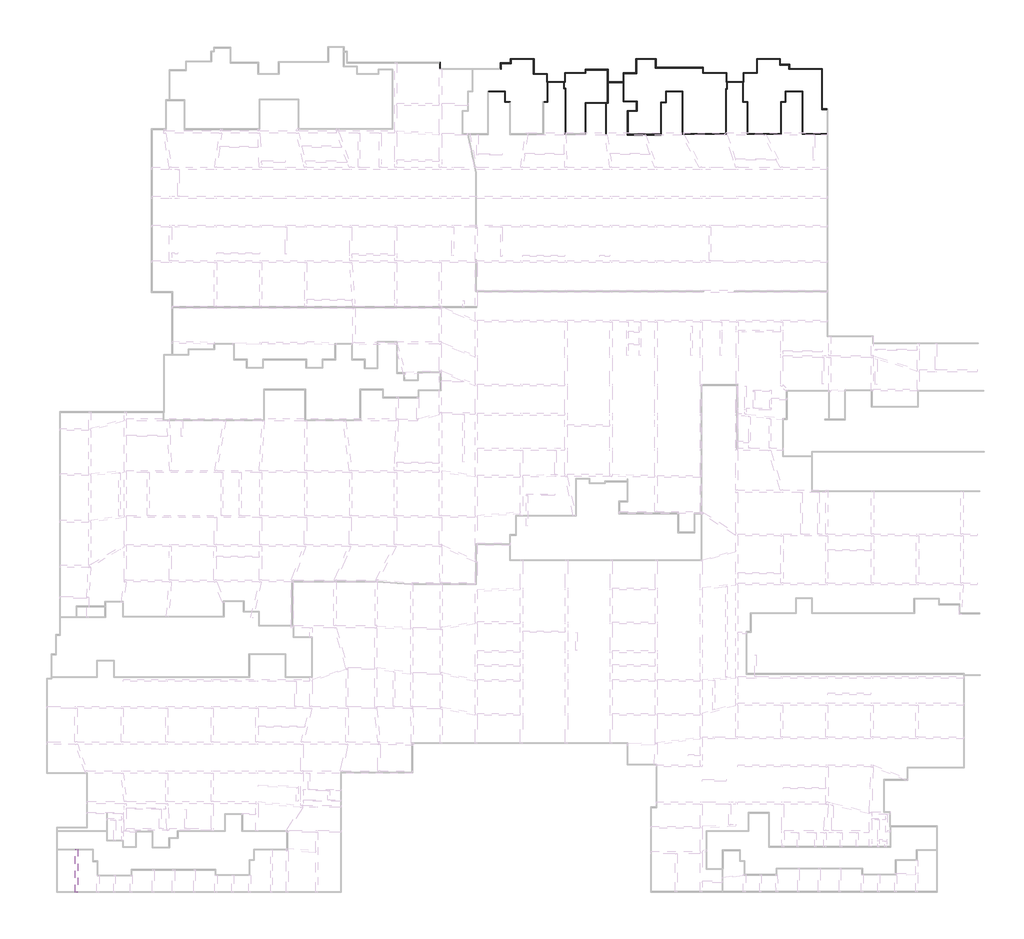
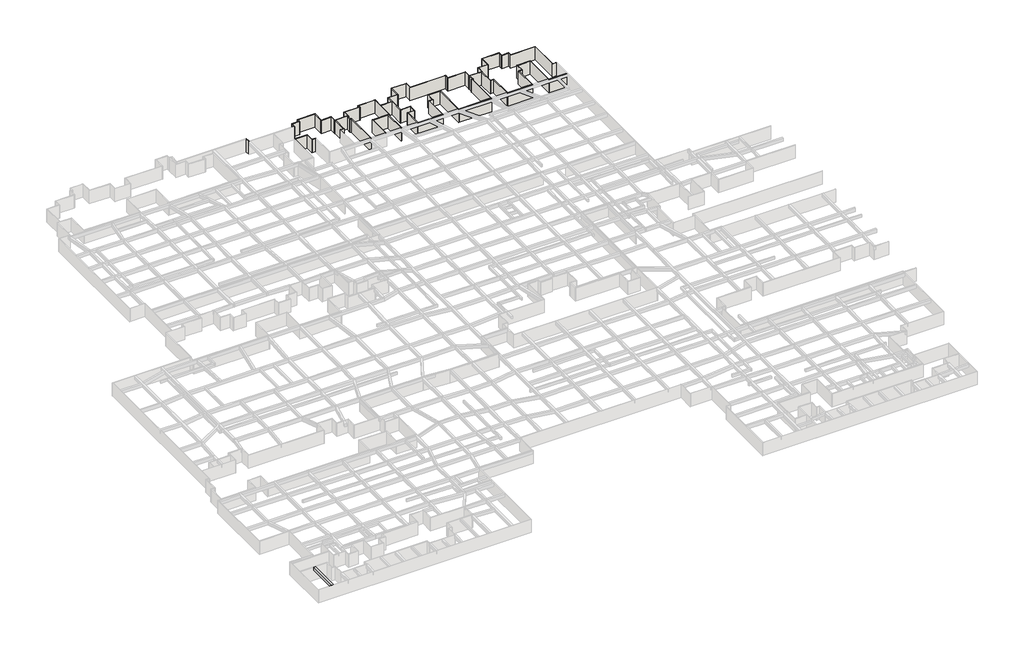
# One storey, part 5 of 16: 70 walls, 1 beam.
"""IFC4 building model written with IfcOpenShell, lengths in millimetres."""

import ifcopenshell
import ifcopenshell.guid

model = None  # the IFC model being written
_history = None  # IfcOwnerHistory: only IFC2X3 demands one
_inside = {}  # id of a spatial element -> (the spatial element, [elements in it])
_under = {}  # id of a project, library or spatial element -> (it, [spatial elements below it])
_declared = {}  # id of a project -> (the project, [libraries it declares])
_typed = {}  # id of a type object -> (the type object, [elements of that type])
_made_of = {}  # id of a material, layer set ... -> (it, [elements and type objects made of it])


def new_model(schema):
    """Start an empty IFC model of exactly this schema.

    Asked for "IFC4X3", IfcOpenShell would pick the latest addendum, in which some entities
    have other attributes; the version numbers below select the first issue.
    IFC2X3 requires an IfcOwnerHistory on every rooted entity: one is made here for all.
    """
    global model, _history
    if schema == "IFC4X3":
        model = ifcopenshell.file(schema_version=(4, 3, 0, 0))
    else:
        model = ifcopenshell.file(schema=schema)
    _inside.clear()
    _under.clear()
    _declared.clear()
    _typed.clear()
    _made_of.clear()
    _history = None
    if model.schema == "IFC2X3":
        org = make("IfcOrganization", Name="unknown")
        user = make(
            "IfcPersonAndOrganization",
            ThePerson=make("IfcPerson", FamilyName="unknown"),
            TheOrganization=org,
        )
        app = make(
            "IfcApplication",
            ApplicationDeveloper=org,
            Version="unknown",
            ApplicationFullName="unknown",
            ApplicationIdentifier="unknown",
        )
        _history = make(
            "IfcOwnerHistory",
            OwningUser=user,
            OwningApplication=app,
            ChangeAction="ADDED",
            CreationDate=0,
        )
    return model


def make(cls, **values):
    """One entity of the class cls with the attributes given. An attribute that is None is left unset."""
    return model.create_entity(
        cls, **{name: value for name, value in values.items() if value is not None}
    )


def rooted(cls, **values):
    """An entity with a GlobalId (a new one), such as an element, a storey or a relation."""
    return make(cls, GlobalId=ifcopenshell.guid.new(), OwnerHistory=_history, **values)


def si_unit(unit_type, name, prefix=None):
    """IfcSIUnit, for example si_unit("LENGTHUNIT", "METRE", prefix="MILLI")."""
    return make("IfcSIUnit", UnitType=unit_type, Prefix=prefix, Name=name)


def assignment(units):
    """IfcUnitAssignment: the units of a project."""
    return None if units is None else make("IfcUnitAssignment", Units=units)


def point(xyz):
    """IfcCartesianPoint."""
    return None if xyz is None else make("IfcCartesianPoint", Coordinates=xyz)


def direction(xyz):
    """IfcDirection."""
    return None if xyz is None else make("IfcDirection", DirectionRatios=xyz)


def frame(location, z_axis=None, x_axis=None):
    """IfcAxis2Placement3D, a coordinate frame: its origin and axes. An axis left out is left unset."""
    return make(
        "IfcAxis2Placement3D",
        Location=point(location),
        Axis=direction(z_axis),
        RefDirection=direction(x_axis),
    )


def origin():
    """The frame at (0, 0, 0) with its axes left unset."""
    return frame((0.0, 0.0, 0.0))


def origin_with_axes():
    """The frame at (0, 0, 0) with the z axis (0, 0, 1) and the x axis (1, 0, 0) written out."""
    return frame((0.0, 0.0, 0.0), z_axis=(0.0, 0.0, 1.0), x_axis=(1.0, 0.0, 0.0))


def place(relative_to, where):
    """IfcLocalPlacement: puts the frame where relative to a parent placement (None: the world)."""
    return make(
        "IfcLocalPlacement", PlacementRelTo=relative_to, RelativePlacement=where
    )


def context(
    kind, dimensions, precision=None, world=None, true_north=None, identifier=None
):
    """IfcGeometricRepresentationContext, for example the 3D "Model" context."""
    return make(
        "IfcGeometricRepresentationContext",
        ContextIdentifier=identifier,
        ContextType=kind,
        CoordinateSpaceDimension=dimensions,
        Precision=precision,
        WorldCoordinateSystem=world,
        TrueNorth=true_north,
    )


def project(units=None, contexts=None):
    """IfcProject with its units and contexts."""
    return rooted(
        "IfcProject",
        Name="project",
        RepresentationContexts=contexts,
        UnitsInContext=assignment(units),
    )


def spatial(cls, under=None, at=None, **own):
    """A site, building, storey or space (cls), placed at a placement, below another one or the project."""
    s = rooted(cls, ObjectPlacement=at, **own)
    if under is not None:
        _under.setdefault(under.id(), (under, []))[1].append(s)
    return s


def polyline(points):
    """IfcPolyline through the points."""
    return make("IfcPolyline", Points=[point(p) for p in points])


def outline(outer, holes=None, kind="AREA"):
    """IfcArbitraryClosedProfileDef: a profile drawn as a closed curve; with holes, ...WithVoids."""
    if holes is None:
        return make("IfcArbitraryClosedProfileDef", ProfileType=kind, OuterCurve=outer)
    return make(
        "IfcArbitraryProfileDefWithVoids",
        ProfileType=kind,
        OuterCurve=outer,
        InnerCurves=holes,
    )


def extrude(swept, where, along, depth):
    """IfcExtrudedAreaSolid: the profile swept, set in the frame where, extruded along a direction by depth."""
    return make(
        "IfcExtrudedAreaSolid",
        SweptArea=swept,
        Position=where,
        ExtrudedDirection=direction(along),
        Depth=depth,
    )


def faces_of(points, faces, orient=None, outer=None):
    """IfcFace entities. A face is a list of loops; a loop is a list of indices into points, from 0.

    orient and outer hold one flag for each loop. By default every Orientation is true, the
    first loop of a face is its IfcFaceOuterBound and the others are IfcFaceBound.
    """
    made = []
    for i, loops in enumerate(faces):
        bounds = []
        for j, loop in enumerate(loops):
            is_outer = j == 0 if outer is None else outer[i][j]
            bounds.append(
                make(
                    "IfcFaceOuterBound" if is_outer else "IfcFaceBound",
                    Bound=make("IfcPolyLoop", Polygon=[points[k] for k in loop]),
                    Orientation=True if orient is None else orient[i][j],
                )
            )
        made.append(make("IfcFace", Bounds=bounds))
    return made


def faceted_brep(points, faces, orient=None, outer=None, voids=None):
    """IfcFacetedBrep: a solid bounded by flat faces; with voids (closed shells), ...WithVoids."""
    shared = [point(p) for p in points]
    hull = make("IfcClosedShell", CfsFaces=faces_of(shared, faces, orient, outer))
    if voids is None:
        return make("IfcFacetedBrep", Outer=hull)
    return make(
        "IfcFacetedBrepWithVoids",
        Outer=hull,
        Voids=[
            make(cls, CfsFaces=faces_of(shared, fs, o, b)) for cls, fs, o, b in voids
        ],
    )


def shape(context_of_items, identifier, shape_type, items):
    """IfcShapeRepresentation: the items that make up one representation, for example the "Body"."""
    return make(
        "IfcShapeRepresentation",
        ContextOfItems=context_of_items,
        RepresentationIdentifier=identifier,
        RepresentationType=shape_type,
        Items=items,
    )


def source(mapping_origin, context_of_items, identifier, shape_type, items):
    """IfcRepresentationMap: a shape defined once, which mapped items show again and again."""
    return make(
        "IfcRepresentationMap",
        MappingOrigin=mapping_origin,
        MappedRepresentation=shape(context_of_items, identifier, shape_type, items),
    )


def transform(
    local_origin,
    x_axis=None,
    y_axis=None,
    z_axis=None,
    scale=None,
    scale2=None,
    scale3=None,
    uniform=True,
):
    """IfcCartesianTransformationOperator3D, or its non-uniform kind. x_axis, y_axis, z_axis: its Axis1, 2, 3."""
    if uniform:
        return make(
            "IfcCartesianTransformationOperator3D",
            Axis1=direction(x_axis),
            Axis2=direction(y_axis),
            LocalOrigin=point(local_origin),
            Scale=scale,
            Axis3=direction(z_axis),
        )
    return make(
        "IfcCartesianTransformationOperator3DnonUniform",
        Axis1=direction(x_axis),
        Axis2=direction(y_axis),
        LocalOrigin=point(local_origin),
        Scale=scale,
        Axis3=direction(z_axis),
        Scale2=scale2,
        Scale3=scale3,
    )


def mapped(mapping_source, mapping_target):
    """IfcMappedItem: shows the shape of a source again, moved by a transform."""
    return make(
        "IfcMappedItem", MappingSource=mapping_source, MappingTarget=mapping_target
    )


def made_of(thing, what):
    """Note that an element or type object is made of a material, layer set ...; save() writes the relation."""
    if what is not None:
        _made_of.setdefault(what.id(), (what, []))[1].append(thing)
    return thing


def element(
    cls,
    number,
    at=None,
    inside=None,
    cuts=None,
    type_object=None,
    material=None,
    context=None,
    identifier="Body",
    shape_type=None,
    held_by="IfcProductDefinitionShape",
    body=None,
    shapes=None,
    **own,
):
    """One element of the class cls, such as IfcWall. Its Tag is "e" and its number.

    at: its placement. inside: the storey or other place that contains it. cuts: it is an
    opening in that element (IfcRelVoidsElement). A single representation is given by context,
    identifier, shape_type and body (its items); several are given by shapes. held_by: the class
    of the entity that holds the representations. save() writes the other relations.
    """
    e = rooted(cls, Tag="e%d" % number, ObjectPlacement=at, **own)
    if body is not None:
        shapes = [shape(context, identifier, shape_type, body)]
    if shapes is not None:
        e.Representation = make(held_by, Representations=shapes)
    if inside is not None:
        _inside.setdefault(inside.id(), (inside, []))[1].append(e)
    if cuts is not None:
        rooted(
            "IfcRelVoidsElement", RelatingBuildingElement=cuts, RelatedOpeningElement=e
        )
    if type_object is not None:
        _typed.setdefault(type_object.id(), (type_object, []))[1].append(e)
    return made_of(e, material)


def aggregate(whole, parts):
    """IfcRelAggregates: a whole, such as a stair, and the parts it consists of."""
    return rooted("IfcRelAggregates", RelatingObject=whole, RelatedObjects=parts)


def save(model, path):
    """Write the relations noted so far, then the file.

    IfcRelAggregates (storeys below a building ...), IfcRelContainedInSpatialStructure (elements
    in a storey), IfcRelDefinesByType, IfcRelAssociatesMaterial and IfcRelDeclares: one each for
    every whole, place, type object, material and project.
    """
    for whole, parts in _under.values():
        aggregate(whole, parts)
    for where, things in _inside.values():
        rooted(
            "IfcRelContainedInSpatialStructure",
            RelatedElements=things,
            RelatingStructure=where,
        )
    for kind, things in _typed.values():
        rooted("IfcRelDefinesByType", RelatedObjects=things, RelatingType=kind)
    for what, things in _made_of.values():
        rooted("IfcRelAssociatesMaterial", RelatedObjects=things, RelatingMaterial=what)
    for by, libraries in _declared.values():
        rooted("IfcRelDeclares", RelatingContext=by, RelatedDefinitions=libraries)
    model.write(path)


def kl_beam_eab3c69a(model_context):
    return source(origin(), model_context, "Body", "SweptSolid", [
        extrude(outline(polyline([(3851.0, 200.0), (3851.0, -200.0), (-3851.0, -200.0), (-3851.0, 200.0), (3851.0, 200.0)])), frame((0.0, 0.0, -400.0), z_axis=(0.0, 0.0, 1.0), x_axis=(1.0, 0.0, 0.0)), (0.0, 0.0, 1.0), 800.0),
    ])


model = new_model("IFC4")

# Units and contexts
model_context = context("Model", 3, world=origin())
ifc_project = project(units=[si_unit("LENGTHUNIT", "METRE", prefix="MILLI")], contexts=[model_context])

# Site, building, storey
site = spatial("IfcSite", under=ifc_project)
building = spatial("IfcBuilding", under=site)
storey = spatial("IfcBuildingStorey", under=building, Name="户型图", Elevation=0.0)

# Beam
placement = place(None, origin())
kl_beam_shape = kl_beam_eab3c69a(model_context)
element("IfcBeam", 1, ObjectType="KL_beam", at=placement, inside=storey, context=model_context, shape_type="MappedRepresentation", body=[
    mapped(kl_beam_shape, transform((69597.2422757, 63756.0820134, 2900.0), x_axis=(0.0, 1.0, 0.0), y_axis=(-1.0, 0.0, 0.0), z_axis=(0.0, 0.0, 1.0))),
])

# Walls
element("IfcWall", 2, at=placement, inside=storey, context=model_context, shape_type="Brep", body=[
    faceted_brep([(204566.5546537, 200822.7290951, 0.0), (203726.5546537, 200822.7290951, 0.0), (203606.5546537, 200822.7290951, 0.0), (203606.5546537, 200822.7290951, 3300.0), (203726.5546537, 200822.7290951, 3300.0), (204566.5546537, 200822.7290951, 3300.0), (204566.5546537, 200702.7290951, 0.0), (204566.5546537, 200702.7290951, 3300.0), (203606.5546537, 200702.7290951, 3300.0), (203606.5546537, 200702.7290951, 0.0)], [[[0, 1, 2, 3, 4, 5]], [[6, 7, 8, 9]], [[2, 1, 0, 6, 9]], [[5, 4, 3, 8, 7]], [[0, 5, 7, 6]], [[3, 2, 9, 8]]]),
])
element("IfcWall", 3, at=placement, inside=storey, context=model_context, shape_type="Brep", body=[
    faceted_brep([(203726.5546537, 200822.7290951, 0.0), (203726.5546537, 208022.6509701, 0.0), (203726.5546537, 208022.6509701, 3300.0), (203726.5546537, 200822.7290951, 3300.0), (203606.5546537, 200822.7290951, 0.0), (203606.5546537, 200822.7290951, 3300.0), (203606.5546537, 207902.6509701, 3300.0), (203606.5546537, 208022.6509701, 3300.0), (203606.5546537, 208022.6509701, 0.0), (203606.5546537, 207902.6509701, 0.0)], [[[0, 1, 2, 3]], [[4, 5, 6, 7, 8, 9]], [[1, 0, 4, 9, 8]], [[3, 2, 7, 6, 5]], [[0, 3, 5, 4]], [[2, 1, 8, 7]]]),
])
element("IfcWall", 4, at=placement, inside=storey, context=model_context, shape_type="Brep", body=[
    faceted_brep([(203606.5546537, 208022.6509701, 0.0), (197813.5060859, 208022.6509701, 0.0), (197693.5060859, 208022.6509701, 0.0), (197693.5060859, 208022.6509701, 3300.0), (197813.5060859, 208022.6509701, 3300.0), (203606.5546537, 208022.6509701, 3300.0), (203606.5546537, 207902.6509701, 0.0), (203606.5546537, 207902.6509701, 3300.0), (197693.5060859, 207902.6509701, 3300.0), (197693.5060859, 207902.6509701, 0.0)], [[[0, 1, 2, 3, 4, 5]], [[6, 7, 8, 9]], [[2, 1, 0, 6, 9]], [[5, 4, 3, 8, 7]], [[0, 5, 7, 6]], [[3, 2, 9, 8]]]),
])
element("IfcWall", 5, at=placement, inside=storey, context=model_context, shape_type="Brep", body=[
    faceted_brep([(197813.5060859, 208022.6509701, 0.0), (197813.5060859, 208822.5710733, 0.0), (197813.5060859, 208822.5710733, 3300.0), (197813.5060859, 208022.6509701, 3300.0), (197693.5060859, 208022.6509701, 0.0), (197693.5060859, 208022.6509701, 3300.0), (197693.5060859, 208702.5710733, 3300.0), (197693.5060859, 208822.5710733, 3300.0), (197693.5060859, 208822.5710733, 0.0), (197693.5060859, 208702.5710733, 0.0)], [[[0, 1, 2, 3]], [[4, 5, 6, 7, 8, 9]], [[1, 0, 4, 9, 8]], [[3, 2, 7, 6, 5]], [[0, 3, 5, 4]], [[2, 1, 8, 7]]]),
])
element("IfcWall", 6, at=placement, inside=storey, context=model_context, shape_type="Brep", body=[
    faceted_brep([(197693.5060859, 208822.5710733, 0.0), (196163.5308894, 208822.5710733, 0.0), (196043.5308894, 208822.5710733, 0.0), (196043.5308894, 208822.5710733, 3300.0), (196163.5308894, 208822.5710733, 3300.0), (197693.5060859, 208822.5710733, 3300.0), (197693.5060859, 208702.5710733, 0.0), (197693.5060859, 208702.5710733, 3300.0), (196043.5308894, 208702.5710733, 3300.0), (196043.5308894, 208702.5710733, 0.0)], [[[0, 1, 2, 3, 4, 5]], [[6, 7, 8, 9]], [[2, 1, 0, 6, 9]], [[5, 4, 3, 8, 7]], [[0, 5, 7, 6]], [[3, 2, 9, 8]]]),
])
element("IfcWall", 7, at=placement, inside=storey, context=model_context, shape_type="Brep", body=[
    faceted_brep([(196163.5308894, 208822.5710733, 0.0), (196163.5308894, 209822.6499935, 0.0), (196163.5308894, 209822.6499935, 3300.0), (196163.5308894, 208822.5710733, 3300.0), (196043.5308894, 208822.5710733, 0.0), (196043.5308894, 208822.5710733, 3300.0), (196043.5308894, 209702.6499935, 3300.0), (196043.5308894, 209822.6499935, 3300.0), (196043.5308894, 209822.6499935, 0.0), (196043.5308894, 209702.6499935, 0.0)], [[[0, 1, 2, 3]], [[4, 5, 6, 7, 8, 9]], [[1, 0, 4, 9, 8]], [[3, 2, 7, 6, 5]], [[0, 3, 5, 4]], [[2, 1, 8, 7]]]),
])
element("IfcWall", 8, at=placement, inside=storey, context=model_context, shape_type="Brep", body=[
    faceted_brep([(196043.5308894, 209822.6499935, 0.0), (191893.5570951, 209822.6499935, 0.0), (191893.5570951, 209822.6499935, 3300.0), (196043.5308894, 209822.6499935, 3300.0), (196043.5308894, 209702.6499935, 0.0), (196043.5308894, 209702.6499935, 3300.0), (192013.5570951, 209702.6499935, 3300.0), (191893.5570951, 209702.6499935, 3300.0), (191893.5570951, 209702.6499935, 0.0), (192013.5570951, 209702.6499935, 0.0)], [[[0, 1, 2, 3]], [[4, 5, 6, 7, 8, 9]], [[1, 0, 4, 9, 8]], [[3, 2, 7, 6, 5]], [[0, 3, 5, 4]], [[2, 1, 8, 7]]]),
])
element("IfcWall", 9, at=placement, inside=storey, context=model_context, shape_type="Brep", body=[
    faceted_brep([(191893.5570951, 209702.6499935, 0.0), (191893.5570951, 207322.6499935, 0.0), (191893.5570951, 207202.6499935, 0.0), (191893.5570951, 207202.6499935, 3300.0), (191893.5570951, 207322.6499935, 3300.0), (191893.5570951, 209702.6499935, 3300.0), (192013.5570951, 209702.6499935, 0.0), (192013.5570951, 209702.6499935, 3300.0), (192013.5570951, 207202.6499935, 3300.0), (192013.5570951, 207202.6499935, 0.0)], [[[0, 1, 2, 3, 4, 5]], [[6, 7, 8, 9]], [[2, 1, 0, 6, 9]], [[5, 4, 3, 8, 7]], [[0, 5, 7, 6]], [[3, 2, 9, 8]]]),
])
element("IfcWall", 10, at=placement, inside=storey, context=model_context, shape_type="Brep", body=[
    faceted_brep([(191893.5570951, 207322.6499935, 0.0), (189493.5570951, 207322.6499935, 0.0), (189493.5570951, 207322.6499935, 3300.0), (191893.5570951, 207322.6499935, 3300.0), (191893.5570951, 207202.6499935, 0.0), (191893.5570951, 207202.6499935, 3300.0), (189613.5570951, 207202.6499935, 3300.0), (189493.5570951, 207202.6499935, 3300.0), (189493.5570951, 207202.6499935, 0.0), (189613.5570951, 207202.6499935, 0.0)], [[[0, 1, 2, 3]], [[4, 5, 6, 7, 8, 9]], [[1, 0, 4, 9, 8]], [[3, 2, 7, 6, 5]], [[0, 3, 5, 4]], [[2, 1, 8, 7]]]),
])
element("IfcWall", 11, at=placement, inside=storey, context=model_context, shape_type="Brep", body=[
    faceted_brep([(189493.5570951, 207202.6499935, 0.0), (189493.5570951, 205722.6499935, 0.0), (189493.5570951, 205602.6499935, 0.0), (189493.5570951, 205602.6499935, 3300.0), (189493.5570951, 205722.6499935, 3300.0), (189493.5570951, 207202.6499935, 3300.0), (189613.5570951, 207202.6499935, 0.0), (189613.5570951, 207202.6499935, 3300.0), (189613.5570951, 205602.6499935, 3300.0), (189613.5570951, 205602.6499935, 0.0)], [[[0, 1, 2, 3, 4, 5]], [[6, 7, 8, 9]], [[2, 1, 0, 6, 9]], [[5, 4, 3, 8, 7]], [[0, 5, 7, 6]], [[3, 2, 9, 8]]]),
])
element("IfcWall", 12, at=placement, inside=storey, context=model_context, shape_type="Brep", body=[
    faceted_brep([(189493.5570951, 205722.6499935, 0.0), (186513.5570951, 205722.6499935, 0.0), (186393.5570951, 205722.6499935, 0.0), (186393.5570951, 205722.6499935, 3300.0), (186513.5570951, 205722.6499935, 3300.0), (189493.5570951, 205722.6499935, 3300.0), (189493.5570951, 205602.6499935, 0.0), (189493.5570951, 205602.6499935, 3300.0), (189373.5570951, 205602.6499935, 3300.0), (186633.5590482, 205602.6499935, 3300.0), (186513.5590482, 205602.6499935, 3300.0), (186393.5570951, 205602.6499935, 3300.0), (186393.5570951, 205602.6499935, 0.0), (186513.5590482, 205602.6499935, 0.0), (186633.5590482, 205602.6499935, 0.0), (189373.5570951, 205602.6499935, 0.0)], [[[0, 1, 2, 3, 4, 5]], [[6, 7, 8, 9, 10, 11, 12, 13, 14, 15]], [[2, 1, 0, 6, 15, 14, 13, 12]], [[5, 4, 3, 11, 10, 9, 8, 7]], [[0, 5, 7, 6]], [[3, 2, 12, 11]]]),
])
element("IfcWall", 13, at=placement, inside=storey, context=model_context, shape_type="Brep", body=[
    faceted_brep([(186513.5570951, 205722.6499935, 0.0), (186513.5570951, 207322.6499935, 0.0), (186513.5570951, 207322.6499935, 3300.0), (186513.5570951, 205722.6499935, 3300.0), (186393.5570951, 205722.6499935, 0.0), (186393.5570951, 205722.6499935, 3300.0), (186393.5570951, 207202.6499935, 3300.0), (186393.5570951, 207322.6499935, 3300.0), (186393.5570951, 207322.6499935, 0.0), (186393.5570951, 207202.6499935, 0.0)], [[[0, 1, 2, 3]], [[4, 5, 6, 7, 8, 9]], [[1, 0, 4, 9, 8]], [[3, 2, 7, 6, 5]], [[0, 3, 5, 4]], [[2, 1, 8, 7]]]),
])
element("IfcWall", 14, at=placement, inside=storey, context=model_context, shape_type="Brep", body=[
    faceted_brep([(186393.5570951, 207322.6499935, 0.0), (182313.5570951, 207322.6499935, 0.0), (182193.5570951, 207322.6499935, 0.0), (182193.5570951, 207322.6499935, 3300.0), (182313.5570951, 207322.6499935, 3300.0), (186393.5570951, 207322.6499935, 3300.0), (186393.5570951, 207202.6499935, 0.0), (186393.5570951, 207202.6499935, 3300.0), (182193.5570951, 207202.6499935, 3300.0), (182193.5570951, 207202.6499935, 0.0)], [[[0, 1, 2, 3, 4, 5]], [[6, 7, 8, 9]], [[2, 1, 0, 6, 9]], [[5, 4, 3, 8, 7]], [[0, 5, 7, 6]], [[3, 2, 9, 8]]]),
])
element("IfcWall", 15, at=placement, inside=storey, context=model_context, shape_type="Brep", body=[
    faceted_brep([(182313.5570951, 207322.6499935, 0.0), (182313.5570951, 208272.6509701, 0.0), (182313.5570951, 208272.6509701, 3300.0), (182313.5570951, 207322.6499935, 3300.0), (182193.5570951, 207322.6499935, 0.0), (182193.5570951, 207322.6499935, 3300.0), (182193.5570951, 208152.6509701, 3300.0), (182193.5570951, 208272.6509701, 3300.0), (182193.5570951, 208272.6509701, 0.0), (182193.5570951, 208152.6509701, 0.0)], [[[0, 1, 2, 3]], [[4, 5, 6, 7, 8, 9]], [[1, 0, 4, 9, 8]], [[3, 2, 7, 6, 5]], [[0, 3, 5, 4]], [[2, 1, 8, 7]]]),
])
element("IfcWall", 16, at=placement, inside=storey, context=model_context, shape_type="Brep", body=[
    faceted_brep([(182193.5570951, 208272.6509701, 0.0), (173813.5570951, 208272.6509701, 0.0), (173693.5570951, 208272.6509701, 0.0), (173693.5570951, 208272.6509701, 3300.0), (173813.5570951, 208272.6509701, 3300.0), (182193.5570951, 208272.6509701, 3300.0), (182193.5570951, 208152.6509701, 0.0), (182193.5570951, 208152.6509701, 3300.0), (173693.5570951, 208152.6509701, 3300.0), (173693.5570951, 208152.6509701, 0.0)], [[[0, 1, 2, 3, 4, 5]], [[6, 7, 8, 9]], [[2, 1, 0, 6, 9]], [[5, 4, 3, 8, 7]], [[0, 5, 7, 6]], [[3, 2, 9, 8]]]),
])
element("IfcWall", 17, at=placement, inside=storey, context=model_context, shape_type="Brep", body=[
    faceted_brep([(173813.5570951, 208272.6509701, 0.0), (173813.5570951, 209872.6509701, 0.0), (173813.5570951, 209872.6509701, 3300.0), (173813.5570951, 208272.6509701, 3300.0), (173693.5570951, 208272.6509701, 0.0), (173693.5570951, 208272.6509701, 3300.0), (173693.5570951, 209752.6509701, 3300.0), (173693.5570951, 209872.6509701, 3300.0), (173693.5570951, 209872.6509701, 0.0), (173693.5570951, 209752.6509701, 0.0)], [[[0, 1, 2, 3]], [[4, 5, 6, 7, 8, 9]], [[1, 0, 4, 9, 8]], [[3, 2, 7, 6, 5]], [[0, 3, 5, 4]], [[2, 1, 8, 7]]]),
])
element("IfcWall", 18, at=placement, inside=storey, context=model_context, shape_type="Brep", body=[
    faceted_brep([(173693.5570951, 209872.6509701, 0.0), (170193.5570951, 209872.6509701, 0.0), (170193.5570951, 209872.6509701, 3300.0), (173693.5570951, 209872.6509701, 3300.0), (173693.5570951, 209752.6509701, 0.0), (173693.5570951, 209752.6509701, 3300.0), (170313.5570951, 209752.6509701, 3300.0), (170193.5570951, 209752.6509701, 3300.0), (170193.5570951, 209752.6509701, 0.0), (170313.5570951, 209752.6509701, 0.0)], [[[0, 1, 2, 3]], [[4, 5, 6, 7, 8, 9]], [[1, 0, 4, 9, 8]], [[3, 2, 7, 6, 5]], [[0, 3, 5, 4]], [[2, 1, 8, 7]]]),
])
element("IfcWall", 19, at=placement, inside=storey, context=model_context, shape_type="Brep", body=[
    faceted_brep([(170193.5570951, 209752.6509701, 0.0), (170193.5570951, 207272.6509701, 0.0), (170193.5570951, 207152.6509701, 0.0), (170193.5570951, 207152.6509701, 3300.0), (170193.5570951, 207272.6509701, 3300.0), (170193.5570951, 209752.6509701, 3300.0), (170313.5570951, 209752.6509701, 0.0), (170313.5570951, 209752.6509701, 3300.0), (170313.5570951, 207152.6509701, 3300.0), (170313.5570951, 207152.6509701, 0.0)], [[[0, 1, 2, 3, 4, 5]], [[6, 7, 8, 9]], [[2, 1, 0, 6, 9]], [[5, 4, 3, 8, 7]], [[0, 5, 7, 6]], [[3, 2, 9, 8]]]),
])
element("IfcWall", 20, at=placement, inside=storey, context=model_context, shape_type="Brep", body=[
    faceted_brep([(170193.5570951, 207272.6509701, 0.0), (167893.5570951, 207272.6509701, 0.0), (167893.5570951, 207272.6509701, 3300.0), (170193.5570951, 207272.6509701, 3300.0), (170193.5570951, 207152.6509701, 0.0), (170193.5570951, 207152.6509701, 3300.0), (168013.5570951, 207152.6509701, 3300.0), (167893.5570951, 207152.6509701, 3300.0), (167893.5570951, 207152.6509701, 0.0), (168013.5570951, 207152.6509701, 0.0)], [[[0, 1, 2, 3]], [[4, 5, 6, 7, 8, 9]], [[1, 0, 4, 9, 8]], [[3, 2, 7, 6, 5]], [[0, 3, 5, 4]], [[2, 1, 8, 7]]]),
])
element("IfcWall", 21, at=placement, inside=storey, context=model_context, shape_type="Brep", body=[
    faceted_brep([(167893.5570951, 207152.6509701, 0.0), (167893.5570951, 205672.6509701, 0.0), (167893.5570951, 205552.6509701, 0.0), (167893.5570951, 202052.6509701, 0.0), (167893.5570951, 202052.6509701, 3300.0), (167893.5570951, 205552.6509701, 3300.0), (167893.5570951, 205672.6509701, 3300.0), (167893.5570951, 207152.6509701, 3300.0), (168013.5570951, 207152.6509701, 0.0), (168013.5570951, 207152.6509701, 3300.0), (168013.5570951, 202172.6509701, 3300.0), (168013.5570951, 202052.6509701, 3300.0), (168013.5570951, 202052.6509701, 0.0), (168013.5570951, 202172.6509701, 0.0)], [[[0, 1, 2, 3, 4, 5, 6, 7]], [[8, 9, 10, 11, 12, 13]], [[3, 2, 1, 0, 8, 13, 12]], [[7, 6, 5, 4, 11, 10, 9]], [[0, 7, 9, 8]], [[4, 3, 12, 11]]]),
])
element("IfcWall", 22, at=placement, inside=storey, context=model_context, shape_type="SweptSolid", body=[
    extrude(outline(polyline([(165183.5551419, 205672.6509701), (167893.5570951, 205672.6509701), (167893.5570951, 205552.6509701), (165183.5551419, 205552.6509701), (165183.5551419, 205672.6509701)])), origin_with_axes(), (0.0, 0.0, 1.0), 3300.0),
])
element("IfcWall", 23, at=placement, inside=storey, context=model_context, shape_type="Brep", body=[
    faceted_brep([(165183.5551419, 201802.6509701, 0.0), (165183.5551419, 205552.6509701, 0.0), (165183.5551419, 205672.6509701, 0.0), (165183.5551419, 207922.6509701, 0.0), (165183.5551419, 207922.6509701, 3300.0), (165183.5551419, 205672.6509701, 3300.0), (165183.5551419, 205552.6509701, 3300.0), (165183.5551419, 201802.6509701, 3300.0), (165063.5551419, 201802.6509701, 0.0), (165063.5551419, 201802.6509701, 3300.0), (165063.5551419, 201922.6509701, 3300.0), (165063.5551419, 207802.6509701, 3300.0), (165063.5551419, 207922.6509701, 3300.0), (165063.5551419, 207922.6509701, 0.0), (165063.5551419, 207802.6509701, 0.0), (165063.5551419, 201922.6509701, 0.0)], [[[0, 1, 2, 3, 4, 5, 6, 7]], [[8, 9, 10, 11, 12, 13, 14, 15]], [[3, 2, 1, 0, 8, 15, 14, 13]], [[7, 6, 5, 4, 12, 11, 10, 9]], [[4, 3, 13, 12]], [[0, 7, 9, 8]]]),
])
element("IfcWall", 24, at=placement, inside=storey, context=model_context, shape_type="Brep", body=[
    faceted_brep([(165063.5551419, 207922.6509701, 0.0), (161063.5551419, 207922.6509701, 0.0), (161063.5551419, 207922.6509701, 3300.0), (165063.5551419, 207922.6509701, 3300.0), (165063.5551419, 207802.6509701, 0.0), (165063.5551419, 207802.6509701, 3300.0), (161183.5551419, 207802.6509701, 3300.0), (161063.5551419, 207802.6509701, 3300.0), (161063.5551419, 207802.6509701, 0.0), (161183.5551419, 207802.6509701, 0.0)], [[[0, 1, 2, 3]], [[4, 5, 6, 7, 8, 9]], [[1, 0, 4, 9, 8]], [[3, 2, 7, 6, 5]], [[0, 3, 5, 4]], [[2, 1, 8, 7]]]),
])
element("IfcWall", 25, at=placement, inside=storey, context=model_context, shape_type="Brep", body=[
    faceted_brep([(161063.5551419, 207802.6509701, 0.0), (161063.5551419, 207322.6509701, 0.0), (161063.5551419, 207202.6509701, 0.0), (161063.5551419, 207202.6509701, 3300.0), (161063.5551419, 207322.6509701, 3300.0), (161063.5551419, 207802.6509701, 3300.0), (161183.5551419, 207802.6509701, 0.0), (161183.5551419, 207802.6509701, 3300.0), (161183.5551419, 207202.6509701, 3300.0), (161183.5551419, 207202.6509701, 0.0)], [[[0, 1, 2, 3, 4, 5]], [[6, 7, 8, 9]], [[2, 1, 0, 6, 9]], [[5, 4, 3, 8, 7]], [[0, 5, 7, 6]], [[3, 2, 9, 8]]]),
])
element("IfcWall", 26, at=placement, inside=storey, context=model_context, shape_type="Brep", body=[
    faceted_brep([(161063.5551419, 207322.6509701, 0.0), (157363.5551419, 207322.6509701, 0.0), (157363.5551419, 207322.6509701, 3300.0), (161063.5551419, 207322.6509701, 3300.0), (161063.5551419, 207202.6509701, 0.0), (161063.5551419, 207202.6509701, 3300.0), (157483.5551419, 207202.6509701, 3300.0), (157363.5551419, 207202.6509701, 3300.0), (157363.5551419, 207202.6509701, 0.0), (157483.5551419, 207202.6509701, 0.0)], [[[0, 1, 2, 3]], [[4, 5, 6, 7, 8, 9]], [[1, 0, 4, 9, 8]], [[3, 2, 7, 6, 5]], [[0, 3, 5, 4]], [[2, 1, 8, 7]]]),
])
element("IfcWall", 27, at=placement, inside=storey, context=model_context, shape_type="Brep", body=[
    faceted_brep([(157363.5551419, 207202.6509701, 0.0), (157363.5551419, 205722.6509701, 0.0), (157363.5551419, 205602.6509701, 0.0), (157363.5551419, 205602.6509701, 3300.0), (157363.5551419, 205722.6509701, 3300.0), (157363.5551419, 207202.6509701, 3300.0), (157483.5551419, 207202.6509701, 0.0), (157483.5551419, 207202.6509701, 3300.0), (157483.5551419, 205602.6509701, 3300.0), (157483.5551419, 205602.6509701, 0.0)], [[[0, 1, 2, 3, 4, 5]], [[6, 7, 8, 9]], [[2, 1, 0, 6, 9]], [[5, 4, 3, 8, 7]], [[0, 5, 7, 6]], [[3, 2, 9, 8]]]),
])
element("IfcWall", 28, at=placement, inside=storey, context=model_context, shape_type="Brep", body=[
    faceted_brep([(157363.5551419, 205722.6509701, 0.0), (154283.5551419, 205722.6509701, 0.0), (154163.5551419, 205722.6509701, 0.0), (154163.5551419, 205722.6509701, 3300.0), (154283.5551419, 205722.6509701, 3300.0), (157363.5551419, 205722.6509701, 3300.0), (157363.5551419, 205602.6509701, 0.0), (157363.5551419, 205602.6509701, 3300.0), (157333.5551419, 205602.6509701, 3300.0), (157213.5551419, 205602.6509701, 3300.0), (154383.5546537, 205602.6509701, 3300.0), (154263.5546537, 205602.6509701, 3300.0), (154163.5551419, 205602.6509701, 3300.0), (154163.5551419, 205602.6509701, 0.0), (154263.5546537, 205602.6509701, 0.0), (154383.5546537, 205602.6509701, 0.0), (157213.5551419, 205602.6509701, 0.0), (157333.5551419, 205602.6509701, 0.0)], [[[0, 1, 2, 3, 4, 5]], [[6, 7, 8, 9, 10, 11, 12, 13, 14, 15, 16, 17]], [[2, 1, 0, 6, 17, 16, 15, 14, 13]], [[5, 4, 3, 12, 11, 10, 9, 8, 7]], [[0, 5, 7, 6]], [[3, 2, 13, 12]]]),
])
element("IfcWall", 29, at=placement, inside=storey, context=model_context, shape_type="Brep", body=[
    faceted_brep([(154283.5551419, 205722.6509701, 0.0), (154283.5551419, 207172.6509701, 0.0), (154283.5551419, 207172.6509701, 3300.0), (154283.5551419, 205722.6509701, 3300.0), (154163.5551419, 205722.6509701, 0.0), (154163.5551419, 205722.6509701, 3300.0), (154163.5551419, 207052.6509701, 3300.0), (154163.5551419, 207172.6509701, 3300.0), (154163.5551419, 207172.6509701, 0.0), (154163.5551419, 207052.6509701, 0.0)], [[[0, 1, 2, 3]], [[4, 5, 6, 7, 8, 9]], [[1, 0, 4, 9, 8]], [[3, 2, 7, 6, 5]], [[0, 3, 5, 4]], [[2, 1, 8, 7]]]),
])
element("IfcWall", 30, at=placement, inside=storey, context=model_context, shape_type="Brep", body=[
    faceted_brep([(154163.5551419, 207172.6509701, 0.0), (151883.5531888, 207172.6509701, 0.0), (151763.5531888, 207172.6509701, 0.0), (151763.5531888, 207172.6509701, 3300.0), (151883.5531888, 207172.6509701, 3300.0), (154163.5551419, 207172.6509701, 3300.0), (154163.5551419, 207052.6509701, 0.0), (154163.5551419, 207052.6509701, 3300.0), (151763.5531888, 207052.6509701, 3300.0), (151763.5531888, 207052.6509701, 0.0)], [[[0, 1, 2, 3, 4, 5]], [[6, 7, 8, 9]], [[2, 1, 0, 6, 9]], [[5, 4, 3, 8, 7]], [[0, 5, 7, 6]], [[3, 2, 9, 8]]]),
])
element("IfcWall", 31, at=placement, inside=storey, context=model_context, shape_type="Brep", body=[
    faceted_brep([(151883.5531888, 207172.6509701, 0.0), (151883.5531888, 209822.6499935, 0.0), (151883.5531888, 209822.6499935, 3300.0), (151883.5531888, 207172.6509701, 3300.0), (151763.5531888, 207172.6509701, 0.0), (151763.5531888, 207172.6509701, 3300.0), (151763.5531888, 209702.6499935, 3300.0), (151763.5531888, 209822.6499935, 3300.0), (151763.5531888, 209822.6499935, 0.0), (151763.5531888, 209702.6499935, 0.0)], [[[0, 1, 2, 3]], [[4, 5, 6, 7, 8, 9]], [[1, 0, 4, 9, 8]], [[3, 2, 7, 6, 5]], [[0, 3, 5, 4]], [[2, 1, 8, 7]]]),
])
element("IfcWall", 32, at=placement, inside=storey, context=model_context, shape_type="Brep", body=[
    faceted_brep([(151763.5531888, 209822.6499935, 0.0), (147613.5451849, 209822.6499935, 0.0), (147613.5451849, 209822.6499935, 3300.0), (151763.5531888, 209822.6499935, 3300.0), (151763.5531888, 209702.6499935, 0.0), (151763.5531888, 209702.6499935, 3300.0), (147733.5451849, 209702.6499935, 3300.0), (147613.5451849, 209702.6499935, 3300.0), (147613.5451849, 209702.6499935, 0.0), (147733.5451849, 209702.6499935, 0.0)], [[[0, 1, 2, 3]], [[4, 5, 6, 7, 8, 9]], [[1, 0, 4, 9, 8]], [[3, 2, 7, 6, 5]], [[0, 3, 5, 4]], [[2, 1, 8, 7]]]),
])
element("IfcWall", 33, at=placement, inside=storey, context=model_context, shape_type="Brep", body=[
    faceted_brep([(147613.5451849, 209702.6499935, 0.0), (147613.5451849, 209072.597906, 0.0), (147613.5451849, 208952.597906, 0.0), (147613.5451849, 208952.597906, 3300.0), (147613.5451849, 209072.597906, 3300.0), (147613.5451849, 209702.6499935, 3300.0), (147733.5451849, 209702.6499935, 0.0), (147733.5451849, 209702.6499935, 3300.0), (147733.5451849, 208952.597906, 3300.0), (147733.5451849, 208952.597906, 0.0)], [[[0, 1, 2, 3, 4, 5]], [[6, 7, 8, 9]], [[2, 1, 0, 6, 9]], [[5, 4, 3, 8, 7]], [[0, 5, 7, 6]], [[3, 2, 9, 8]]]),
])
element("IfcWall", 34, at=placement, inside=storey, context=model_context, shape_type="Brep", body=[
    faceted_brep([(147613.5451849, 209072.597906, 0.0), (145813.5451849, 209072.597906, 0.0), (145813.5451849, 209072.597906, 3300.0), (147613.5451849, 209072.597906, 3300.0), (147613.5451849, 208952.597906, 0.0), (147613.5451849, 208952.597906, 3300.0), (145933.5451849, 208952.597906, 3300.0), (145813.5451849, 208952.597906, 3300.0), (145813.5451849, 208952.597906, 0.0), (145933.5451849, 208952.597906, 0.0)], [[[0, 1, 2, 3]], [[4, 5, 6, 7, 8, 9]], [[1, 0, 4, 9, 8]], [[3, 2, 7, 6, 5]], [[0, 3, 5, 4]], [[2, 1, 8, 7]]]),
])
element("IfcWall", 35, at=placement, inside=storey, context=model_context, shape_type="Brep", body=[
    faceted_brep([(145813.5451849, 208952.597906, 0.0), (145813.5451849, 208022.6509701, 0.0), (145813.5451849, 207902.6509701, 0.0), (145813.5451849, 207902.6509701, 3300.0), (145813.5451849, 208022.6509701, 3300.0), (145813.5451849, 208952.597906, 3300.0), (145933.5451849, 208952.597906, 0.0), (145933.5451849, 208952.597906, 3300.0), (145933.5451849, 207902.6509701, 3300.0), (145933.5451849, 207902.6509701, 0.0)], [[[0, 1, 2, 3, 4, 5]], [[6, 7, 8, 9]], [[2, 1, 0, 6, 9]], [[5, 4, 3, 8, 7]], [[0, 5, 7, 6]], [[3, 2, 9, 8]]]),
])
element("IfcWall", 36, at=placement, inside=storey, context=model_context, shape_type="Brep", body=[
    faceted_brep([(135026.242901, 208022.6509701, 0.0), (135026.242901, 209172.8384701, 0.0), (135026.242901, 209172.8384701, 3300.0), (135026.242901, 208022.6509701, 3300.0), (134906.242901, 208022.6509701, 0.0), (134906.242901, 208022.6509701, 3300.0), (134906.242901, 209052.8384701, 3300.0), (134906.242901, 209172.8384701, 3300.0), (134906.242901, 209172.8384701, 0.0), (134906.242901, 209052.8384701, 0.0)], [[[0, 1, 2, 3]], [[4, 5, 6, 7, 8, 9]], [[1, 0, 4, 9, 8]], [[3, 2, 7, 6, 5]], [[0, 3, 5, 4]], [[2, 1, 8, 7]]]),
])
element("IfcWall", 37, at=placement, inside=storey, context=model_context, shape_type="Brep", body=[
    faceted_brep([(143683.5664576, 203907.301294, 0.0), (146563.5546537, 203907.301294, 0.0), (146683.5546537, 203907.301294, 0.0), (146683.5546537, 203907.301294, 3300.0), (146563.5546537, 203907.301294, 3300.0), (143683.5664576, 203907.301294, 3300.0), (143683.5664576, 204027.301294, 0.0), (143683.5664576, 204027.301294, 3300.0), (146683.5546537, 204027.301294, 3300.0), (146683.5546537, 204027.301294, 0.0)], [[[0, 1, 2, 3, 4, 5]], [[6, 7, 8, 9]], [[2, 1, 0, 6, 9]], [[5, 4, 3, 8, 7]], [[0, 5, 7, 6]], [[3, 2, 9, 8]]]),
])
element("IfcWall", 38, at=placement, inside=storey, context=model_context, shape_type="Brep", body=[
    faceted_brep([(146563.5546537, 203907.301294, 0.0), (146563.5546537, 202007.301294, 0.0), (146563.5546537, 202007.301294, 3300.0), (146563.5546537, 203907.301294, 3300.0), (146683.5546537, 203907.301294, 0.0), (146683.5546537, 203907.301294, 3300.0), (146683.5546537, 202127.301294, 3300.0), (146683.5546537, 202007.301294, 3300.0), (146683.5546537, 202007.301294, 0.0), (146683.5546537, 202127.301294, 0.0)], [[[0, 1, 2, 3]], [[4, 5, 6, 7, 8, 9]], [[1, 0, 4, 9, 8]], [[3, 2, 7, 6, 5]], [[0, 3, 5, 4]], [[2, 1, 8, 7]]]),
])
element("IfcWall", 39, at=placement, inside=storey, context=model_context, shape_type="Brep", body=[
    faceted_brep([(146683.5546537, 202007.301294, 0.0), (147463.5546537, 202007.301294, 0.0), (147583.5546537, 202007.301294, 0.0), (147583.5546537, 202007.301294, 3300.0), (147463.5546537, 202007.301294, 3300.0), (146683.5546537, 202007.301294, 3300.0), (146683.5546537, 202127.301294, 0.0), (146683.5546537, 202127.301294, 3300.0), (147583.5546537, 202127.301294, 3300.0), (147583.5546537, 202127.301294, 0.0)], [[[0, 1, 2, 3, 4, 5]], [[6, 7, 8, 9]], [[2, 1, 0, 6, 9]], [[5, 4, 3, 8, 7]], [[0, 5, 7, 6]], [[3, 2, 9, 8]]]),
])
element("IfcWall", 40, at=placement, inside=storey, context=model_context, shape_type="Brep", body=[
    faceted_brep([(153583.5546537, 202007.301294, 0.0), (154383.5546537, 202007.301294, 0.0), (154383.5546537, 202007.301294, 3300.0), (153583.5546537, 202007.301294, 3300.0), (153583.5546537, 202127.301294, 0.0), (153583.5546537, 202127.301294, 3300.0), (154263.5546537, 202127.301294, 3300.0), (154383.5546537, 202127.301294, 3300.0), (154383.5546537, 202127.301294, 0.0), (154263.5546537, 202127.301294, 0.0)], [[[0, 1, 2, 3]], [[4, 5, 6, 7, 8, 9]], [[1, 0, 4, 9, 8]], [[3, 2, 7, 6, 5]], [[0, 3, 5, 4]], [[2, 1, 8, 7]]]),
])
element("IfcWall", 41, at=placement, inside=storey, context=model_context, shape_type="SweptSolid", body=[
    extrude(outline(polyline([(154383.5546537, 205602.6509701), (154383.5546537, 202127.301294), (154263.5546537, 202127.301294), (154263.5546537, 205602.6509701), (154383.5546537, 205602.6509701)])), origin_with_axes(), (0.0, 0.0, 1.0), 3300.0),
])
element("IfcWall", 42, at=placement, inside=storey, context=model_context, shape_type="SweptSolid", body=[
    extrude(outline(polyline([(157213.5551419, 204522.6509701), (157213.5551419, 205602.6509701), (157333.5551419, 205602.6509701), (157333.5551419, 204522.6509701), (157213.5551419, 204522.6509701)])), origin_with_axes(), (0.0, 0.0, 1.0), 3300.0),
])
element("IfcWall", 43, at=placement, inside=storey, context=model_context, shape_type="Brep", body=[
    faceted_brep([(157213.5551419, 204402.6509701, 0.0), (157463.5564847, 204402.6509701, 0.0), (157583.5564847, 204402.6509701, 0.0), (157583.5564847, 204402.6509701, 3300.0), (157463.5564847, 204402.6509701, 3300.0), (157213.5551419, 204402.6509701, 3300.0), (157213.5551419, 204522.6509701, 0.0), (157213.5551419, 204522.6509701, 3300.0), (157333.5551419, 204522.6509701, 3300.0), (157583.5564847, 204522.6509701, 3300.0), (157583.5564847, 204522.6509701, 0.0), (157333.5551419, 204522.6509701, 0.0)], [[[0, 1, 2, 3, 4, 5]], [[6, 7, 8, 9, 10, 11]], [[2, 1, 0, 6, 11, 10]], [[5, 4, 3, 9, 8, 7]], [[0, 5, 7, 6]], [[3, 2, 10, 9]]]),
])
element("IfcWall", 44, at=placement, inside=storey, context=model_context, shape_type="Brep", body=[
    faceted_brep([(157463.5564847, 204402.6509701, 0.0), (157463.5564847, 196202.6509701, 0.0), (157463.5564847, 196202.6509701, 3300.0), (157463.5564847, 204402.6509701, 3300.0), (157583.5564847, 204402.6509701, 0.0), (157583.5564847, 204402.6509701, 3300.0), (157583.5564847, 196322.6509701, 3300.0), (157583.5564847, 196202.6509701, 3300.0), (157583.5564847, 196202.6509701, 0.0), (157583.5564847, 196322.6509701, 0.0)], [[[0, 1, 2, 3]], [[4, 5, 6, 7, 8, 9]], [[1, 0, 4, 9, 8]], [[3, 2, 7, 6, 5]], [[0, 3, 5, 4]], [[2, 1, 8, 7]]]),
])
element("IfcWall", 45, at=placement, inside=storey, context=model_context, shape_type="Brep", body=[
    faceted_brep([(161183.5564847, 196322.6509701, 0.0), (161183.5564847, 201802.6509701, 0.0), (161183.5564847, 201922.6509701, 0.0), (161183.5564847, 201922.6509701, 3300.0), (161183.5564847, 201802.6509701, 3300.0), (161183.5564847, 196322.6509701, 3300.0), (161063.5564847, 196322.6509701, 0.0), (161063.5564847, 196322.6509701, 3300.0), (161063.5564847, 201922.6509701, 3300.0), (161063.5564847, 201922.6509701, 0.0)], [[[0, 1, 2, 3, 4, 5]], [[6, 7, 8, 9]], [[2, 1, 0, 6, 9]], [[5, 4, 3, 8, 7]], [[0, 5, 7, 6]], [[3, 2, 9, 8]]]),
])
element("IfcWall", 46, at=placement, inside=storey, context=model_context, shape_type="Brep", body=[
    faceted_brep([(161183.5564847, 201802.6509701, 0.0), (164763.5564847, 201802.6509701, 0.0), (164883.5564847, 201802.6509701, 0.0), (165063.5551419, 201802.6509701, 0.0), (165063.5551419, 201802.6509701, 3300.0), (164883.5564847, 201802.6509701, 3300.0), (164763.5564847, 201802.6509701, 3300.0), (161183.5564847, 201802.6509701, 3300.0), (161183.5564847, 201922.6509701, 0.0), (161183.5564847, 201922.6509701, 3300.0), (165063.5551419, 201922.6509701, 3300.0), (165063.5551419, 201922.6509701, 0.0)], [[[0, 1, 2, 3, 4, 5, 6, 7]], [[8, 9, 10, 11]], [[3, 2, 1, 0, 8, 11]], [[7, 6, 5, 4, 10, 9]], [[0, 7, 9, 8]], [[4, 3, 11, 10]]]),
])
element("IfcWall", 47, at=placement, inside=storey, context=model_context, shape_type="SweptSolid", body=[
    extrude(outline(polyline([(164763.5564847, 196362.6509701), (164763.5564847, 201802.6509701), (164883.5564847, 201802.6509701), (164883.5564847, 196362.6509701), (164763.5564847, 196362.6509701)])), origin_with_axes(), (0.0, 0.0, 1.0), 3300.0),
])
element("IfcWall", 48, at=placement, inside=storey, context=model_context, shape_type="Brep", body=[
    faceted_brep([(168013.5570951, 202052.6509701, 0.0), (170293.5570951, 202052.6509701, 0.0), (170413.5570951, 202052.6509701, 0.0), (170413.5570951, 202052.6509701, 3300.0), (170293.5570951, 202052.6509701, 3300.0), (168013.5570951, 202052.6509701, 3300.0), (168013.5570951, 202172.6509701, 0.0), (168013.5570951, 202172.6509701, 3300.0), (170413.5570951, 202172.6509701, 3300.0), (170413.5570951, 202172.6509701, 0.0)], [[[0, 1, 2, 3, 4, 5]], [[6, 7, 8, 9]], [[2, 1, 0, 6, 9]], [[5, 4, 3, 8, 7]], [[0, 5, 7, 6]], [[3, 2, 9, 8]]]),
])
element("IfcWall", 49, at=placement, inside=storey, context=model_context, shape_type="Brep", body=[
    faceted_brep([(170293.5570951, 202052.6509701, 0.0), (170293.5570951, 200522.5610928, 0.0), (170293.5570951, 200402.5610928, 0.0), (170293.5570951, 200402.5610928, 3300.0), (170293.5570951, 200522.5610928, 3300.0), (170293.5570951, 202052.6509701, 3300.0), (170413.5570951, 202052.6509701, 0.0), (170413.5570951, 202052.6509701, 3300.0), (170413.5570951, 200402.5610928, 3300.0), (170413.5570951, 200402.5610928, 0.0)], [[[0, 1, 2, 3, 4, 5]], [[6, 7, 8, 9]], [[2, 1, 0, 6, 9]], [[5, 4, 3, 8, 7]], [[0, 5, 7, 6]], [[3, 2, 9, 8]]]),
])
element("IfcWall", 50, at=placement, inside=storey, context=model_context, shape_type="Brep", body=[
    faceted_brep([(170293.5570951, 200522.5610928, 0.0), (168662.7526059, 200522.5610928, 0.0), (168662.7526059, 200522.5610928, 3300.0), (170293.5570951, 200522.5610928, 3300.0), (170293.5570951, 200402.5610928, 0.0), (170293.5570951, 200402.5610928, 3300.0), (168782.7526059, 200402.5610928, 3300.0), (168662.7526059, 200402.5610928, 3300.0), (168662.7526059, 200402.5610928, 0.0), (168782.7526059, 200402.5610928, 0.0)], [[[0, 1, 2, 3]], [[4, 5, 6, 7, 8, 9]], [[1, 0, 4, 9, 8]], [[3, 2, 7, 6, 5]], [[0, 3, 5, 4]], [[2, 1, 8, 7]]]),
])
element("IfcWall", 51, at=placement, inside=storey, context=model_context, shape_type="Brep", body=[
    faceted_brep([(168662.7526059, 200402.5610928, 0.0), (168662.7526059, 196102.7447201, 0.0), (168662.7526059, 196102.7447201, 3300.0), (168662.7526059, 200402.5610928, 3300.0), (168782.7526059, 200402.5610928, 0.0), (168782.7526059, 200402.5610928, 3300.0), (168782.7526059, 196222.7447201, 3300.0), (168782.7526059, 196102.7447201, 3300.0), (168782.7526059, 196102.7447201, 0.0), (168782.7526059, 196222.7447201, 0.0)], [[[0, 1, 2, 3]], [[4, 5, 6, 7, 8, 9]], [[1, 0, 4, 9, 8]], [[3, 2, 7, 6, 5]], [[0, 3, 5, 4]], [[2, 1, 8, 7]]]),
])
element("IfcWall", 52, at=placement, inside=storey, context=model_context, shape_type="Brep", body=[
    faceted_brep([(168782.7526059, 196102.7447201, 0.0), (174782.7526059, 196102.7447201, 0.0), (174782.7526059, 196102.7447201, 3300.0), (168782.7526059, 196102.7447201, 3300.0), (168782.7526059, 196222.7447201, 0.0), (168782.7526059, 196222.7447201, 3300.0), (174662.7526059, 196222.7447201, 3300.0), (174782.7526059, 196222.7447201, 3300.0), (174782.7526059, 196222.7447201, 0.0), (174662.7526059, 196222.7447201, 0.0)], [[[0, 1, 2, 3]], [[4, 5, 6, 7, 8, 9]], [[1, 0, 4, 9, 8]], [[3, 2, 7, 6, 5]], [[0, 3, 5, 4]], [[2, 1, 8, 7]]]),
])
element("IfcWall", 53, at=placement, inside=storey, context=model_context, shape_type="Brep", body=[
    faceted_brep([(174782.7526059, 196222.7447201, 0.0), (174782.7526059, 201902.6509701, 0.0), (174782.7526059, 202022.6509701, 0.0), (174782.7526059, 202022.6509701, 3300.0), (174782.7526059, 201902.6509701, 3300.0), (174782.7526059, 196222.7447201, 3300.0), (174662.7526059, 196222.7447201, 0.0), (174662.7526059, 196222.7447201, 3300.0), (174662.7526059, 202022.6509701, 3300.0), (174662.7526059, 202022.6509701, 0.0)], [[[0, 1, 2, 3, 4, 5]], [[6, 7, 8, 9]], [[2, 1, 0, 6, 9]], [[5, 4, 3, 8, 7]], [[0, 5, 7, 6]], [[3, 2, 9, 8]]]),
])
element("IfcWall", 54, at=placement, inside=storey, context=model_context, shape_type="Brep", body=[
    faceted_brep([(174782.7526059, 201902.6509701, 0.0), (175683.5570951, 201902.6509701, 0.0), (175683.5570951, 201902.6509701, 3300.0), (174782.7526059, 201902.6509701, 3300.0), (174782.7526059, 202022.6509701, 0.0), (174782.7526059, 202022.6509701, 3300.0), (175563.5570951, 202022.6509701, 3300.0), (175683.5570951, 202022.6509701, 3300.0), (175683.5570951, 202022.6509701, 0.0), (175563.5570951, 202022.6509701, 0.0)], [[[0, 1, 2, 3]], [[4, 5, 6, 7, 8, 9]], [[1, 0, 4, 9, 8]], [[3, 2, 7, 6, 5]], [[0, 3, 5, 4]], [[2, 1, 8, 7]]]),
])
element("IfcWall", 55, at=placement, inside=storey, context=model_context, shape_type="Brep", body=[
    faceted_brep([(175683.5570951, 202022.6509701, 0.0), (175683.5570951, 203902.6509701, 0.0), (175683.5570951, 204022.6509701, 0.0), (175683.5570951, 204022.6509701, 3300.0), (175683.5570951, 203902.6509701, 3300.0), (175683.5570951, 202022.6509701, 3300.0), (175563.5570951, 202022.6509701, 0.0), (175563.5570951, 202022.6509701, 3300.0), (175563.5570951, 204022.6509701, 3300.0), (175563.5570951, 204022.6509701, 0.0)], [[[0, 1, 2, 3, 4, 5]], [[6, 7, 8, 9]], [[2, 1, 0, 6, 9]], [[5, 4, 3, 8, 7]], [[0, 5, 7, 6]], [[3, 2, 9, 8]]]),
])
element("IfcWall", 56, at=placement, inside=storey, context=model_context, shape_type="Brep", body=[
    faceted_brep([(175683.5570951, 203902.6509701, 0.0), (178513.5590482, 203902.6509701, 0.0), (178633.5590482, 203902.6509701, 0.0), (178633.5590482, 203902.6509701, 3300.0), (178513.5590482, 203902.6509701, 3300.0), (175683.5570951, 203902.6509701, 3300.0), (175683.5570951, 204022.6509701, 0.0), (175683.5570951, 204022.6509701, 3300.0), (178633.5590482, 204022.6509701, 3300.0), (178633.5590482, 204022.6509701, 0.0)], [[[0, 1, 2, 3, 4, 5]], [[6, 7, 8, 9]], [[2, 1, 0, 6, 9]], [[5, 4, 3, 8, 7]], [[0, 5, 7, 6]], [[3, 2, 9, 8]]]),
])
element("IfcWall", 57, at=placement, inside=storey, context=model_context, shape_type="Brep", body=[
    faceted_brep([(178513.5590482, 203902.6509701, 0.0), (178513.5590482, 196227.561337, 0.0), (178513.5590482, 196227.561337, 3300.0), (178513.5590482, 203902.6509701, 3300.0), (178633.5590482, 203902.6509701, 0.0), (178633.5590482, 203902.6509701, 3300.0), (178633.5590482, 196347.561337, 3300.0), (178633.5590482, 196227.561337, 3300.0), (178633.5590482, 196227.561337, 0.0), (178633.5590482, 196347.561337, 0.0)], [[[0, 1, 2, 3]], [[4, 5, 6, 7, 8, 9]], [[1, 0, 4, 9, 8]], [[3, 2, 7, 6, 5]], [[0, 3, 5, 4]], [[2, 1, 8, 7]]]),
])
element("IfcWall", 58, at=placement, inside=storey, context=model_context, shape_type="Brep", body=[
    faceted_brep([(178633.5590482, 196227.561337, 0.0), (186433.5590482, 196227.561337, 0.0), (186433.5590482, 196227.561337, 3300.0), (178633.5590482, 196227.561337, 3300.0), (178633.5590482, 196347.561337, 0.0), (178633.5590482, 196347.561337, 3300.0), (186313.5590482, 196347.561337, 3300.0), (186433.5590482, 196347.561337, 3300.0), (186433.5590482, 196347.561337, 0.0), (186313.5590482, 196347.561337, 0.0)], [[[0, 1, 2, 3]], [[4, 5, 6, 7, 8, 9]], [[1, 0, 4, 9, 8]], [[3, 2, 7, 6, 5]], [[0, 3, 5, 4]], [[2, 1, 8, 7]]]),
])
element("IfcWall", 59, at=placement, inside=storey, context=model_context, shape_type="SweptSolid", body=[
    extrude(outline(polyline([(186433.5590482, 204327.561337), (186433.5590482, 196347.561337), (186313.5590482, 196347.561337), (186313.5590482, 204327.561337), (186433.5590482, 204327.561337)])), origin_with_axes(), (0.0, 0.0, 1.0), 3300.0),
])
element("IfcWall", 60, at=placement, inside=storey, context=model_context, shape_type="Brep", body=[
    faceted_brep([(186313.5590482, 204327.561337, 0.0), (186433.5590482, 204327.561337, 0.0), (186633.5590482, 204327.561337, 0.0), (186633.5590482, 204327.561337, 3300.0), (186433.5590482, 204327.561337, 3300.0), (186313.5590482, 204327.561337, 3300.0), (186313.5590482, 204447.561337, 0.0), (186313.5590482, 204447.561337, 3300.0), (186513.5590482, 204447.561337, 3300.0), (186633.5590482, 204447.561337, 3300.0), (186633.5590482, 204447.561337, 0.0), (186513.5590482, 204447.561337, 0.0)], [[[0, 1, 2, 3, 4, 5]], [[6, 7, 8, 9, 10, 11]], [[2, 1, 0, 6, 11, 10]], [[5, 4, 3, 9, 8, 7]], [[0, 5, 7, 6]], [[3, 2, 10, 9]]]),
])
element("IfcWall", 61, at=placement, inside=storey, context=model_context, shape_type="SweptSolid", body=[
    extrude(outline(polyline([(186633.5590482, 205602.6499935), (186633.5590482, 204447.561337), (186513.5590482, 204447.561337), (186513.5590482, 205602.6499935), (186633.5590482, 205602.6499935)])), origin_with_axes(), (0.0, 0.0, 1.0), 3300.0),
])
element("IfcWall", 62, at=placement, inside=storey, context=model_context, shape_type="Brep", body=[
    faceted_brep([(189373.5570951, 205602.6499935, 0.0), (189373.5570951, 201982.6499935, 0.0), (189373.5570951, 201982.6499935, 3300.0), (189373.5570951, 205602.6499935, 3300.0), (189493.5570951, 205602.6499935, 0.0), (189493.5570951, 205602.6499935, 3300.0), (189493.5570951, 202102.6499935, 3300.0), (189493.5570951, 201982.6499935, 3300.0), (189493.5570951, 201982.6499935, 0.0), (189493.5570951, 202102.6499935, 0.0)], [[[0, 1, 2, 3]], [[4, 5, 6, 7, 8, 9]], [[1, 0, 4, 9, 8]], [[3, 2, 7, 6, 5]], [[0, 3, 5, 4]], [[2, 1, 8, 7]]]),
])
element("IfcWall", 63, at=placement, inside=storey, context=model_context, shape_type="Brep", body=[
    faceted_brep([(189493.5570951, 201982.6499935, 0.0), (190192.7611504, 201982.6499935, 0.0), (190312.7611504, 201982.6499935, 0.0), (190312.7611504, 201982.6499935, 3300.0), (190192.7611504, 201982.6499935, 3300.0), (189493.5570951, 201982.6499935, 3300.0), (189493.5570951, 202102.6499935, 0.0), (189493.5570951, 202102.6499935, 3300.0), (190312.7611504, 202102.6499935, 3300.0), (190312.7611504, 202102.6499935, 0.0)], [[[0, 1, 2, 3, 4, 5]], [[6, 7, 8, 9]], [[2, 1, 0, 6, 9]], [[5, 4, 3, 8, 7]], [[0, 5, 7, 6]], [[3, 2, 9, 8]]]),
])
element("IfcWall", 64, at=placement, inside=storey, context=model_context, shape_type="Brep", body=[
    faceted_brep([(190192.7611504, 201982.6499935, 0.0), (190192.7611504, 196227.561337, 0.0), (190192.7611504, 196227.561337, 3300.0), (190192.7611504, 201982.6499935, 3300.0), (190312.7611504, 201982.6499935, 0.0), (190312.7611504, 201982.6499935, 3300.0), (190312.7611504, 196347.561337, 3300.0), (190312.7611504, 196227.561337, 3300.0), (190312.7611504, 196227.561337, 0.0), (190312.7611504, 196347.561337, 0.0)], [[[0, 1, 2, 3]], [[4, 5, 6, 7, 8, 9]], [[1, 0, 4, 9, 8]], [[3, 2, 7, 6, 5]], [[0, 3, 5, 4]], [[2, 1, 8, 7]]]),
])
element("IfcWall", 65, at=placement, inside=storey, context=model_context, shape_type="Brep", body=[
    faceted_brep([(190312.7611504, 196227.561337, 0.0), (196326.5590225, 196227.561337, 0.0), (196326.5590225, 196227.561337, 3300.0), (190312.7611504, 196227.561337, 3300.0), (190312.7611504, 196347.561337, 0.0), (190312.7611504, 196347.561337, 3300.0), (196206.5590225, 196347.561337, 3300.0), (196326.5590225, 196347.561337, 3300.0), (196326.5590225, 196347.561337, 0.0), (196206.5590225, 196347.561337, 0.0)], [[[0, 1, 2, 3]], [[4, 5, 6, 7, 8, 9]], [[1, 0, 4, 9, 8]], [[3, 2, 7, 6, 5]], [[0, 3, 5, 4]], [[2, 1, 8, 7]]]),
])
element("IfcWall", 66, at=placement, inside=storey, context=model_context, shape_type="Brep", body=[
    faceted_brep([(196326.5590225, 196347.561337, 0.0), (196326.5590225, 201982.6499935, 0.0), (196326.5590225, 202102.6499935, 0.0), (196326.5590225, 202102.6499935, 3300.0), (196326.5590225, 201982.6499935, 3300.0), (196326.5590225, 196347.561337, 3300.0), (196206.5590225, 196347.561337, 0.0), (196206.5590225, 196347.561337, 3300.0), (196206.5590225, 202102.6499935, 3300.0), (196206.5590225, 202102.6499935, 0.0)], [[[0, 1, 2, 3, 4, 5]], [[6, 7, 8, 9]], [[2, 1, 0, 6, 9]], [[5, 4, 3, 8, 7]], [[0, 5, 7, 6]], [[3, 2, 9, 8]]]),
])
element("IfcWall", 67, at=placement, inside=storey, context=model_context, shape_type="Brep", body=[
    faceted_brep([(196326.5590225, 201982.6499935, 0.0), (197126.5599273, 201982.6499935, 0.0), (197126.5599273, 201982.6499935, 3300.0), (196326.5590225, 201982.6499935, 3300.0), (196326.5590225, 202102.6499935, 0.0), (196326.5590225, 202102.6499935, 3300.0), (197006.5599273, 202102.6499935, 3300.0), (197126.5599273, 202102.6499935, 3300.0), (197126.5599273, 202102.6499935, 0.0), (197006.5599273, 202102.6499935, 0.0)], [[[0, 1, 2, 3]], [[4, 5, 6, 7, 8, 9]], [[1, 0, 4, 9, 8]], [[3, 2, 7, 6, 5]], [[0, 3, 5, 4]], [[2, 1, 8, 7]]]),
])
element("IfcWall", 68, at=placement, inside=storey, context=model_context, shape_type="Brep", body=[
    faceted_brep([(197126.5599273, 202102.6499935, 0.0), (197126.5599273, 203882.6499935, 0.0), (197126.5599273, 204002.6499935, 0.0), (197126.5599273, 204002.6499935, 3300.0), (197126.5599273, 203882.6499935, 3300.0), (197126.5599273, 202102.6499935, 3300.0), (197006.5599273, 202102.6499935, 0.0), (197006.5599273, 202102.6499935, 3300.0), (197006.5599273, 204002.6499935, 3300.0), (197006.5599273, 204002.6499935, 0.0)], [[[0, 1, 2, 3, 4, 5]], [[6, 7, 8, 9]], [[2, 1, 0, 6, 9]], [[5, 4, 3, 8, 7]], [[0, 5, 7, 6]], [[3, 2, 9, 8]]]),
])
element("IfcWall", 69, at=placement, inside=storey, context=model_context, shape_type="Brep", body=[
    faceted_brep([(197126.5599273, 203882.6499935, 0.0), (200106.5599273, 203882.6499935, 0.0), (200226.5599273, 203882.6499935, 0.0), (200226.5599273, 203882.6499935, 3300.0), (200106.5599273, 203882.6499935, 3300.0), (197126.5599273, 203882.6499935, 3300.0), (197126.5599273, 204002.6499935, 0.0), (197126.5599273, 204002.6499935, 3300.0), (200226.5599273, 204002.6499935, 3300.0), (200226.5599273, 204002.6499935, 0.0)], [[[0, 1, 2, 3, 4, 5]], [[6, 7, 8, 9]], [[2, 1, 0, 6, 9]], [[5, 4, 3, 8, 7]], [[0, 5, 7, 6]], [[3, 2, 9, 8]]]),
])
element("IfcWall", 70, at=placement, inside=storey, context=model_context, shape_type="Brep", body=[
    faceted_brep([(200106.5599273, 203882.6499935, 0.0), (200106.5599273, 196227.561337, 0.0), (200106.5599273, 196227.561337, 3300.0), (200106.5599273, 203882.6499935, 3300.0), (200226.5599273, 203882.6499935, 0.0), (200226.5599273, 203882.6499935, 3300.0), (200226.5599273, 196347.561337, 3300.0), (200226.5599273, 196227.561337, 3300.0), (200226.5599273, 196227.561337, 0.0), (200226.5599273, 196347.561337, 0.0)], [[[0, 1, 2, 3]], [[4, 5, 6, 7, 8, 9]], [[1, 0, 4, 9, 8]], [[3, 2, 7, 6, 5]], [[0, 3, 5, 4]], [[2, 1, 8, 7]]]),
])
element("IfcWall", 71, at=placement, inside=storey, context=model_context, shape_type="SweptSolid", body=[
    extrude(outline(polyline([(204566.5546537, 196227.561337), (200226.5599273, 196227.561337), (200226.5599273, 196347.561337), (204566.5546537, 196347.561337), (204566.5546537, 196227.561337)])), origin_with_axes(), (0.0, 0.0, 1.0), 3300.0),
])

save(model, "model.ifc")
